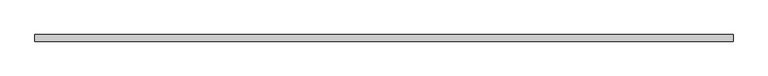
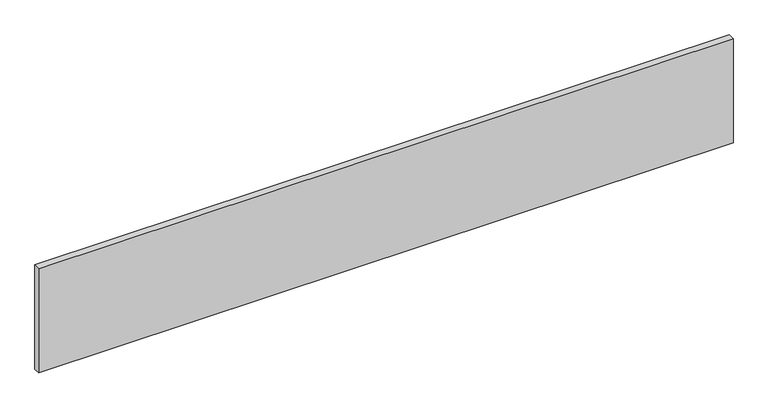
"""IFC4 building model written with IfcOpenShell, lengths in millimetres: proxy geometry, Plywood026 3357 : Plywood026 3357."""

from ifc_helpers import new_model, si_unit, frame, origin, place, context, project, spatial, polyline, outline, extrude, source, transform, mapped, element, save


def generic_models_f6638959(model_context):
    return source(origin(), model_context, "Body", "SweptSolid", [
        extrude(outline(polyline([(3694.2883192, 10214.5258229), (3694.2883192, 10233.5750834), (5694.2883192, 10233.5750834), (5694.2883192, 10214.5258229), (3694.2883192, 10214.5258229)])), frame((0.0, 0.0, 39420.5476563), z_axis=(0.0, 0.0, 1.0), x_axis=(1.0, 0.0, 0.0)), (0.0, 0.0, 1.0), 317.5008096),
    ])


if __name__ == "__main__":
    model = new_model("IFC4")
    model_context = context("Model", 3, world=origin())
    ifc_project = project(units=[si_unit("LENGTHUNIT", "METRE", prefix="MILLI")], contexts=[model_context])
    site = spatial("IfcSite", under=ifc_project)
    building = spatial("IfcBuilding", under=site)
    placement = place(None, origin())
    generic_models_shape = generic_models_f6638959(model_context)
    element("IfcBuildingElementProxy", 1, Name="Plywood026 3357 : Plywood026 3357", ObjectType="Plywood026 3357 : Plywood026 3357", at=placement, inside=building, context=model_context, shape_type="MappedRepresentation", body=[
        mapped(generic_models_shape, transform((0.0, 0.0, 0.0), x_axis=(1.0, 0.0, 0.0), y_axis=(0.0, 1.0, 0.0), z_axis=(0.0, 0.0, 1.0))),
    ])
    save(model, "model.ifc")

# Revit data of these elements
# Type "Plywood026 3357 : Plywood026 3357"
#   NameOverride = "Plywood026"
# Element 1 (IfcBuildingElementProxy, "Plywood026 3357 : Plywood026 3357")
#   Materials on its faces: "CDX PLYWOOD -  SEE STRUCTURAL DWGS"
# Materials
#   "CDX PLYWOOD -  SEE STRUCTURAL DWGS": class "Unassigned", colour RGB 177 130 114, transparency 0, Cost = 0
